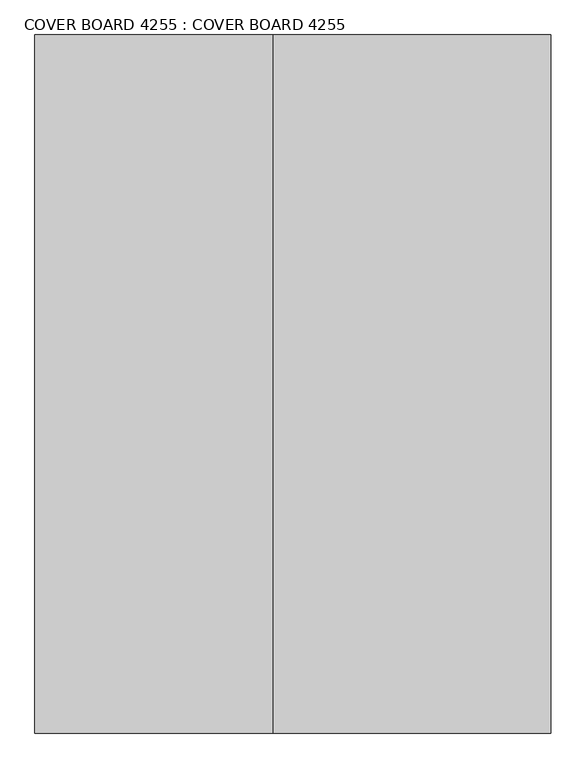
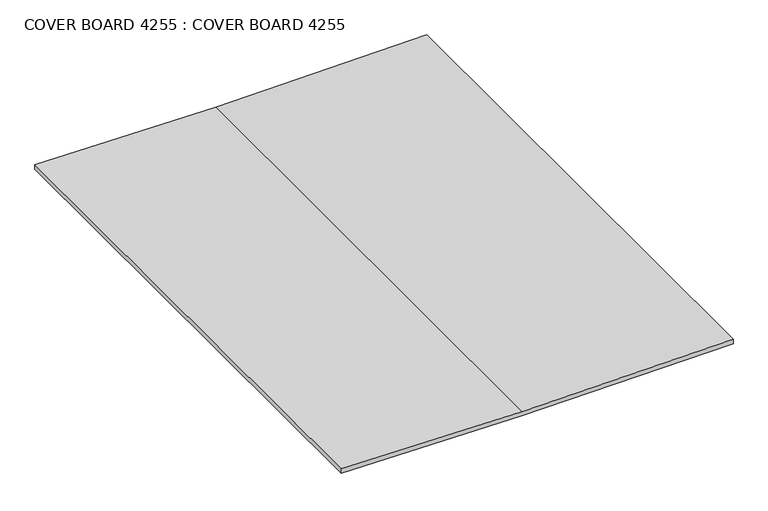
"""IFC4 building model written with IfcOpenShell, lengths in millimetres: proxy geometry, COVER BOARD 4255 : COVER BOARD 4255."""

import ifcopenshell
import ifcopenshell.guid

model = None  # the IFC model being written
_history = None  # IfcOwnerHistory: only IFC2X3 demands one
_inside = {}  # id of a spatial element -> (the spatial element, [elements in it])
_under = {}  # id of a project, library or spatial element -> (it, [spatial elements below it])
_declared = {}  # id of a project -> (the project, [libraries it declares])
_typed = {}  # id of a type object -> (the type object, [elements of that type])
_made_of = {}  # id of a material, layer set ... -> (it, [elements and type objects made of it])


def new_model(schema):
    """Start an empty IFC model of exactly this schema.

    Asked for "IFC4X3", IfcOpenShell would pick the latest addendum, in which some entities
    have other attributes; the version numbers below select the first issue.
    IFC2X3 requires an IfcOwnerHistory on every rooted entity: one is made here for all.
    """
    global model, _history
    if schema == "IFC4X3":
        model = ifcopenshell.file(schema_version=(4, 3, 0, 0))
    else:
        model = ifcopenshell.file(schema=schema)
    _inside.clear()
    _under.clear()
    _declared.clear()
    _typed.clear()
    _made_of.clear()
    _history = None
    if model.schema == "IFC2X3":
        org = make("IfcOrganization", Name="unknown")
        user = make(
            "IfcPersonAndOrganization",
            ThePerson=make("IfcPerson", FamilyName="unknown"),
            TheOrganization=org,
        )
        app = make(
            "IfcApplication",
            ApplicationDeveloper=org,
            Version="unknown",
            ApplicationFullName="unknown",
            ApplicationIdentifier="unknown",
        )
        _history = make(
            "IfcOwnerHistory",
            OwningUser=user,
            OwningApplication=app,
            ChangeAction="ADDED",
            CreationDate=0,
        )
    return model


def make(cls, **values):
    """One entity of the class cls with the attributes given. An attribute that is None is left unset."""
    return model.create_entity(
        cls, **{name: value for name, value in values.items() if value is not None}
    )


def rooted(cls, **values):
    """An entity with a GlobalId (a new one), such as an element, a storey or a relation."""
    return make(cls, GlobalId=ifcopenshell.guid.new(), OwnerHistory=_history, **values)


def si_unit(unit_type, name, prefix=None):
    """IfcSIUnit, for example si_unit("LENGTHUNIT", "METRE", prefix="MILLI")."""
    return make("IfcSIUnit", UnitType=unit_type, Prefix=prefix, Name=name)


def assignment(units):
    """IfcUnitAssignment: the units of a project."""
    return None if units is None else make("IfcUnitAssignment", Units=units)


def point(xyz):
    """IfcCartesianPoint."""
    return None if xyz is None else make("IfcCartesianPoint", Coordinates=xyz)


def direction(xyz):
    """IfcDirection."""
    return None if xyz is None else make("IfcDirection", DirectionRatios=xyz)


def frame(location, z_axis=None, x_axis=None):
    """IfcAxis2Placement3D, a coordinate frame: its origin and axes. An axis left out is left unset."""
    return make(
        "IfcAxis2Placement3D",
        Location=point(location),
        Axis=direction(z_axis),
        RefDirection=direction(x_axis),
    )


def origin():
    """The frame at (0, 0, 0) with its axes left unset."""
    return frame((0.0, 0.0, 0.0))


def place(relative_to, where):
    """IfcLocalPlacement: puts the frame where relative to a parent placement (None: the world)."""
    return make(
        "IfcLocalPlacement", PlacementRelTo=relative_to, RelativePlacement=where
    )


def context(
    kind, dimensions, precision=None, world=None, true_north=None, identifier=None
):
    """IfcGeometricRepresentationContext, for example the 3D "Model" context."""
    return make(
        "IfcGeometricRepresentationContext",
        ContextIdentifier=identifier,
        ContextType=kind,
        CoordinateSpaceDimension=dimensions,
        Precision=precision,
        WorldCoordinateSystem=world,
        TrueNorth=true_north,
    )


def project(units=None, contexts=None):
    """IfcProject with its units and contexts."""
    return rooted(
        "IfcProject",
        Name="project",
        RepresentationContexts=contexts,
        UnitsInContext=assignment(units),
    )


def spatial(cls, under=None, at=None, **own):
    """A site, building, storey or space (cls), placed at a placement, below another one or the project."""
    s = rooted(cls, ObjectPlacement=at, **own)
    if under is not None:
        _under.setdefault(under.id(), (under, []))[1].append(s)
    return s


def polyline(points):
    """IfcPolyline through the points."""
    return make("IfcPolyline", Points=[point(p) for p in points])


def outline(outer, holes=None, kind="AREA"):
    """IfcArbitraryClosedProfileDef: a profile drawn as a closed curve; with holes, ...WithVoids."""
    if holes is None:
        return make("IfcArbitraryClosedProfileDef", ProfileType=kind, OuterCurve=outer)
    return make(
        "IfcArbitraryProfileDefWithVoids",
        ProfileType=kind,
        OuterCurve=outer,
        InnerCurves=holes,
    )


def extrude(swept, where, along, depth):
    """IfcExtrudedAreaSolid: the profile swept, set in the frame where, extruded along a direction by depth."""
    return make(
        "IfcExtrudedAreaSolid",
        SweptArea=swept,
        Position=where,
        ExtrudedDirection=direction(along),
        Depth=depth,
    )


def shape(context_of_items, identifier, shape_type, items):
    """IfcShapeRepresentation: the items that make up one representation, for example the "Body"."""
    return make(
        "IfcShapeRepresentation",
        ContextOfItems=context_of_items,
        RepresentationIdentifier=identifier,
        RepresentationType=shape_type,
        Items=items,
    )


def source(mapping_origin, context_of_items, identifier, shape_type, items):
    """IfcRepresentationMap: a shape defined once, which mapped items show again and again."""
    return make(
        "IfcRepresentationMap",
        MappingOrigin=mapping_origin,
        MappedRepresentation=shape(context_of_items, identifier, shape_type, items),
    )


def transform(
    local_origin,
    x_axis=None,
    y_axis=None,
    z_axis=None,
    scale=None,
    scale2=None,
    scale3=None,
    uniform=True,
):
    """IfcCartesianTransformationOperator3D, or its non-uniform kind. x_axis, y_axis, z_axis: its Axis1, 2, 3."""
    if uniform:
        return make(
            "IfcCartesianTransformationOperator3D",
            Axis1=direction(x_axis),
            Axis2=direction(y_axis),
            LocalOrigin=point(local_origin),
            Scale=scale,
            Axis3=direction(z_axis),
        )
    return make(
        "IfcCartesianTransformationOperator3DnonUniform",
        Axis1=direction(x_axis),
        Axis2=direction(y_axis),
        LocalOrigin=point(local_origin),
        Scale=scale,
        Axis3=direction(z_axis),
        Scale2=scale2,
        Scale3=scale3,
    )


def mapped(mapping_source, mapping_target):
    """IfcMappedItem: shows the shape of a source again, moved by a transform."""
    return make(
        "IfcMappedItem", MappingSource=mapping_source, MappingTarget=mapping_target
    )


def made_of(thing, what):
    """Note that an element or type object is made of a material, layer set ...; save() writes the relation."""
    if what is not None:
        _made_of.setdefault(what.id(), (what, []))[1].append(thing)
    return thing


def element(
    cls,
    number,
    at=None,
    inside=None,
    cuts=None,
    type_object=None,
    material=None,
    context=None,
    identifier="Body",
    shape_type=None,
    held_by="IfcProductDefinitionShape",
    body=None,
    shapes=None,
    **own,
):
    """One element of the class cls, such as IfcWall. Its Tag is "e" and its number.

    at: its placement. inside: the storey or other place that contains it. cuts: it is an
    opening in that element (IfcRelVoidsElement). A single representation is given by context,
    identifier, shape_type and body (its items); several are given by shapes. held_by: the class
    of the entity that holds the representations. save() writes the other relations.
    """
    e = rooted(cls, Tag="e%d" % number, ObjectPlacement=at, **own)
    if body is not None:
        shapes = [shape(context, identifier, shape_type, body)]
    if shapes is not None:
        e.Representation = make(held_by, Representations=shapes)
    if inside is not None:
        _inside.setdefault(inside.id(), (inside, []))[1].append(e)
    if cuts is not None:
        rooted(
            "IfcRelVoidsElement", RelatingBuildingElement=cuts, RelatedOpeningElement=e
        )
    if type_object is not None:
        _typed.setdefault(type_object.id(), (type_object, []))[1].append(e)
    return made_of(e, material)


def aggregate(whole, parts):
    """IfcRelAggregates: a whole, such as a stair, and the parts it consists of."""
    return rooted("IfcRelAggregates", RelatingObject=whole, RelatedObjects=parts)


def save(model, path):
    """Write the relations noted so far, then the file.

    IfcRelAggregates (storeys below a building ...), IfcRelContainedInSpatialStructure (elements
    in a storey), IfcRelDefinesByType, IfcRelAssociatesMaterial and IfcRelDeclares: one each for
    every whole, place, type object, material and project.
    """
    for whole, parts in _under.values():
        aggregate(whole, parts)
    for where, things in _inside.values():
        rooted(
            "IfcRelContainedInSpatialStructure",
            RelatedElements=things,
            RelatingStructure=where,
        )
    for kind, things in _typed.values():
        rooted("IfcRelDefinesByType", RelatedObjects=things, RelatingType=kind)
    for what, things in _made_of.values():
        rooted("IfcRelAssociatesMaterial", RelatedObjects=things, RelatingMaterial=what)
    for by, libraries in _declared.values():
        rooted("IfcRelDeclares", RelatingContext=by, RelatedDefinitions=libraries)
    model.write(path)


def cover_board_4255_cover_board_4255_a2131a35(model_context):
    return source(origin(), model_context, "Body", "SweptSolid", [
        extrude(outline(polyline([(40228.1021556, -1886.5629484), (40237.9000089, -2567.3737014), (40220.5682898, -2567.3737014), (40210.7704365, -1886.5629484), (40220.5682898, -1090.0815411), (40237.9000089, -1090.0815411), (40228.1021556, -1886.5629484)])), frame((0.0, -1052.6406573, 0.0), z_axis=(0.0, 1.0, 0.0), x_axis=(0.0, 0.0, 1.0)), (0.0, 0.0, 1.0), 2000.0),
    ])


if __name__ == "__main__":
    model = new_model("IFC4")
    model_context = context("Model", 3, world=origin())
    ifc_project = project(units=[si_unit("LENGTHUNIT", "METRE", prefix="MILLI")], contexts=[model_context])
    site = spatial("IfcSite", under=ifc_project)
    building = spatial("IfcBuilding", under=site)
    placement = place(None, origin())
    cover_board_4255_cover_board_4255_shape = cover_board_4255_cover_board_4255_a2131a35(model_context)
    element("IfcBuildingElementProxy", 1, Name="COVER BOARD 4255 : COVER BOARD 4255", ObjectType="COVER BOARD 4255 : COVER BOARD 4255", at=placement, inside=building, context=model_context, shape_type="MappedRepresentation", body=[
        mapped(cover_board_4255_cover_board_4255_shape, transform((0.0, 0.0, 0.0), x_axis=(1.0, 0.0, 0.0), y_axis=(0.0, 1.0, 0.0), z_axis=(0.0, 0.0, 1.0))),
    ])
    save(model, "model.ifc")

# Revit data of these elements
# Type "COVER BOARD 4255 : COVER BOARD 4255"
#   NameOverride = "COVER BOARD"
# Element 1 (IfcBuildingElementProxy, "COVER BOARD 4255 : COVER BOARD 4255")
#   Materials on its faces: "CDX PLYWOOD - SEE STRUCTURAL DWGS"
# Materials
#   "CDX PLYWOOD - SEE STRUCTURAL DWGS": class "Unassigned", colour RGB 177 130 114, transparency 0, Cost = 0
